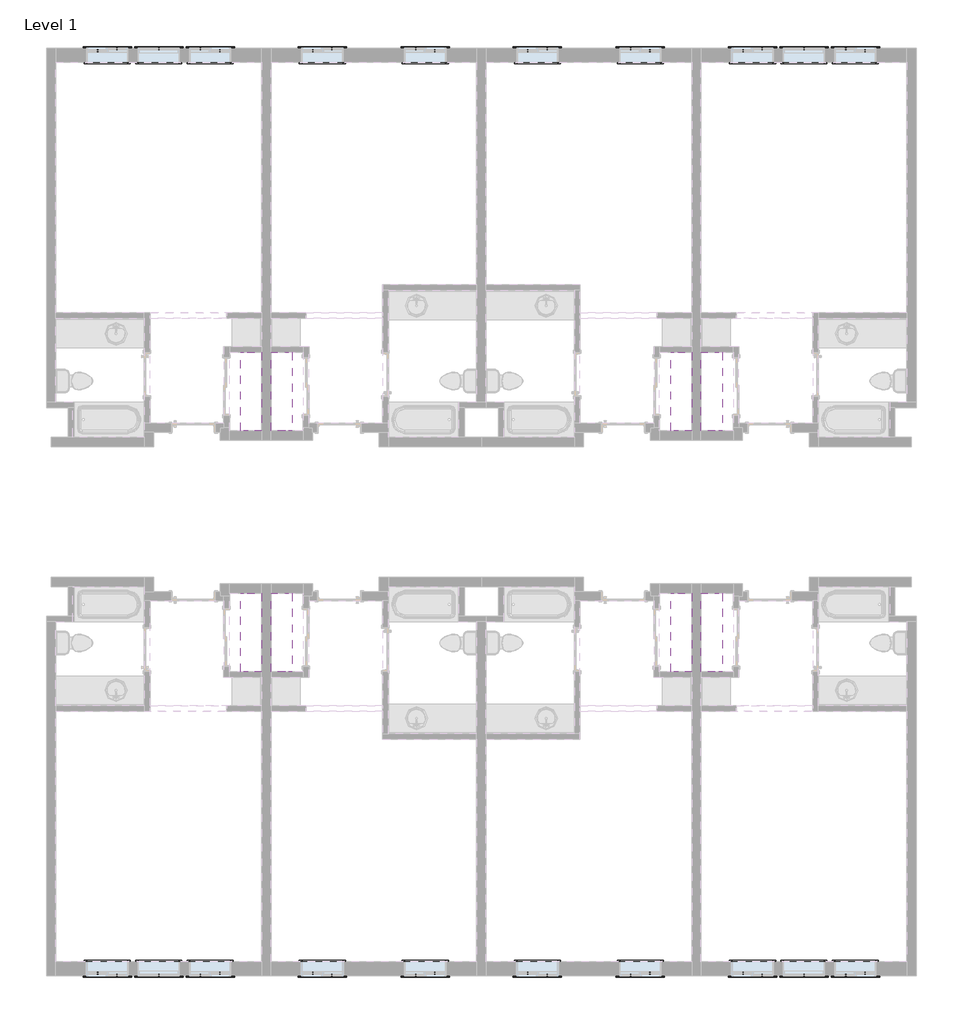
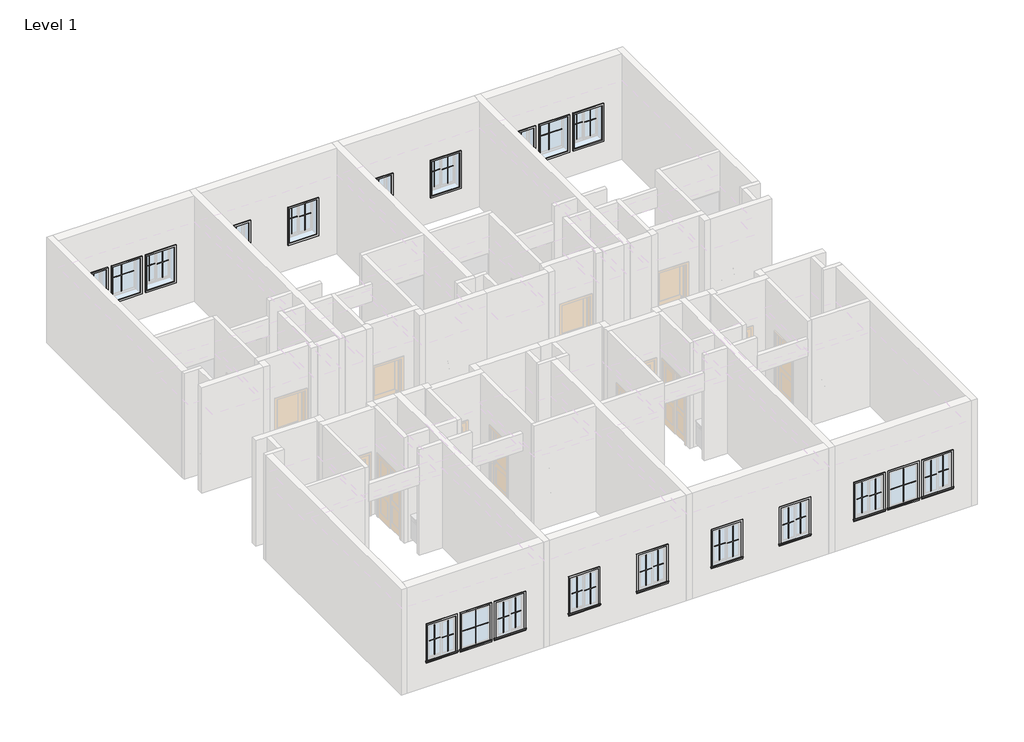
# One storey, part 5 of 5: 84 proxies.
"""IFC4 building model written with IfcOpenShell, lengths in millimetres."""

import ifcopenshell
import ifcopenshell.guid

model = None  # the IFC model being written
_history = None  # IfcOwnerHistory: only IFC2X3 demands one
_inside = {}  # id of a spatial element -> (the spatial element, [elements in it])
_under = {}  # id of a project, library or spatial element -> (it, [spatial elements below it])
_declared = {}  # id of a project -> (the project, [libraries it declares])
_typed = {}  # id of a type object -> (the type object, [elements of that type])
_made_of = {}  # id of a material, layer set ... -> (it, [elements and type objects made of it])


def new_model(schema):
    """Start an empty IFC model of exactly this schema.

    Asked for "IFC4X3", IfcOpenShell would pick the latest addendum, in which some entities
    have other attributes; the version numbers below select the first issue.
    IFC2X3 requires an IfcOwnerHistory on every rooted entity: one is made here for all.
    """
    global model, _history
    if schema == "IFC4X3":
        model = ifcopenshell.file(schema_version=(4, 3, 0, 0))
    else:
        model = ifcopenshell.file(schema=schema)
    _inside.clear()
    _under.clear()
    _declared.clear()
    _typed.clear()
    _made_of.clear()
    _history = None
    if model.schema == "IFC2X3":
        org = make("IfcOrganization", Name="unknown")
        user = make(
            "IfcPersonAndOrganization",
            ThePerson=make("IfcPerson", FamilyName="unknown"),
            TheOrganization=org,
        )
        app = make(
            "IfcApplication",
            ApplicationDeveloper=org,
            Version="unknown",
            ApplicationFullName="unknown",
            ApplicationIdentifier="unknown",
        )
        _history = make(
            "IfcOwnerHistory",
            OwningUser=user,
            OwningApplication=app,
            ChangeAction="ADDED",
            CreationDate=0,
        )
    return model


def make(cls, **values):
    """One entity of the class cls with the attributes given. An attribute that is None is left unset."""
    return model.create_entity(
        cls, **{name: value for name, value in values.items() if value is not None}
    )


def rooted(cls, **values):
    """An entity with a GlobalId (a new one), such as an element, a storey or a relation."""
    return make(cls, GlobalId=ifcopenshell.guid.new(), OwnerHistory=_history, **values)


def si_unit(unit_type, name, prefix=None):
    """IfcSIUnit, for example si_unit("LENGTHUNIT", "METRE", prefix="MILLI")."""
    return make("IfcSIUnit", UnitType=unit_type, Prefix=prefix, Name=name)


def assignment(units):
    """IfcUnitAssignment: the units of a project."""
    return None if units is None else make("IfcUnitAssignment", Units=units)


def point(xyz):
    """IfcCartesianPoint."""
    return None if xyz is None else make("IfcCartesianPoint", Coordinates=xyz)


def direction(xyz):
    """IfcDirection."""
    return None if xyz is None else make("IfcDirection", DirectionRatios=xyz)


def frame(location, z_axis=None, x_axis=None):
    """IfcAxis2Placement3D, a coordinate frame: its origin and axes. An axis left out is left unset."""
    return make(
        "IfcAxis2Placement3D",
        Location=point(location),
        Axis=direction(z_axis),
        RefDirection=direction(x_axis),
    )


def frame_2d(location, x_axis=None):
    """IfcAxis2Placement2D, a coordinate frame in the plane: its origin and x axis."""
    return make(
        "IfcAxis2Placement2D", Location=point(location), RefDirection=direction(x_axis)
    )


def origin():
    """The frame at (0, 0, 0) with its axes left unset."""
    return frame((0.0, 0.0, 0.0))


def origin_with_axes():
    """The frame at (0, 0, 0) with the z axis (0, 0, 1) and the x axis (1, 0, 0) written out."""
    return frame((0.0, 0.0, 0.0), z_axis=(0.0, 0.0, 1.0), x_axis=(1.0, 0.0, 0.0))


def place(relative_to, where):
    """IfcLocalPlacement: puts the frame where relative to a parent placement (None: the world)."""
    return make(
        "IfcLocalPlacement", PlacementRelTo=relative_to, RelativePlacement=where
    )


def context(
    kind, dimensions, precision=None, world=None, true_north=None, identifier=None
):
    """IfcGeometricRepresentationContext, for example the 3D "Model" context."""
    return make(
        "IfcGeometricRepresentationContext",
        ContextIdentifier=identifier,
        ContextType=kind,
        CoordinateSpaceDimension=dimensions,
        Precision=precision,
        WorldCoordinateSystem=world,
        TrueNorth=true_north,
    )


def project(units=None, contexts=None):
    """IfcProject with its units and contexts."""
    return rooted(
        "IfcProject",
        Name="project",
        RepresentationContexts=contexts,
        UnitsInContext=assignment(units),
    )


def spatial(cls, under=None, at=None, **own):
    """A site, building, storey or space (cls), placed at a placement, below another one or the project."""
    s = rooted(cls, ObjectPlacement=at, **own)
    if under is not None:
        _under.setdefault(under.id(), (under, []))[1].append(s)
    return s


def polyline(points):
    """IfcPolyline through the points."""
    return make("IfcPolyline", Points=[point(p) for p in points])


def circle_curve(where, radius):
    """IfcCircle in the frame where."""
    return make("IfcCircle", Position=where, Radius=radius)


def trimmed(basis, trim1, trim2, sense, master):
    """IfcTrimmedCurve: the piece of a basis curve between two trims."""
    return make(
        "IfcTrimmedCurve",
        BasisCurve=basis,
        Trim1=trim1,
        Trim2=trim2,
        SenseAgreement=sense,
        MasterRepresentation=master,
    )


def segment(curve, same_sense, transition):
    """IfcCompositeCurveSegment."""
    return make(
        "IfcCompositeCurveSegment",
        Transition=transition,
        SameSense=same_sense,
        ParentCurve=curve,
    )


def composite_curve(segments, self_intersect=None):
    """IfcCompositeCurve: segments joined end to end."""
    return make("IfcCompositeCurve", Segments=segments, SelfIntersect=self_intersect)


def outline(outer, holes=None, kind="AREA"):
    """IfcArbitraryClosedProfileDef: a profile drawn as a closed curve; with holes, ...WithVoids."""
    if holes is None:
        return make("IfcArbitraryClosedProfileDef", ProfileType=kind, OuterCurve=outer)
    return make(
        "IfcArbitraryProfileDefWithVoids",
        ProfileType=kind,
        OuterCurve=outer,
        InnerCurves=holes,
    )


def extrude(swept, where, along, depth):
    """IfcExtrudedAreaSolid: the profile swept, set in the frame where, extruded along a direction by depth."""
    return make(
        "IfcExtrudedAreaSolid",
        SweptArea=swept,
        Position=where,
        ExtrudedDirection=direction(along),
        Depth=depth,
    )


def shape(context_of_items, identifier, shape_type, items):
    """IfcShapeRepresentation: the items that make up one representation, for example the "Body"."""
    return make(
        "IfcShapeRepresentation",
        ContextOfItems=context_of_items,
        RepresentationIdentifier=identifier,
        RepresentationType=shape_type,
        Items=items,
    )


def source(mapping_origin, context_of_items, identifier, shape_type, items):
    """IfcRepresentationMap: a shape defined once, which mapped items show again and again."""
    return make(
        "IfcRepresentationMap",
        MappingOrigin=mapping_origin,
        MappedRepresentation=shape(context_of_items, identifier, shape_type, items),
    )


def transform(
    local_origin,
    x_axis=None,
    y_axis=None,
    z_axis=None,
    scale=None,
    scale2=None,
    scale3=None,
    uniform=True,
):
    """IfcCartesianTransformationOperator3D, or its non-uniform kind. x_axis, y_axis, z_axis: its Axis1, 2, 3."""
    if uniform:
        return make(
            "IfcCartesianTransformationOperator3D",
            Axis1=direction(x_axis),
            Axis2=direction(y_axis),
            LocalOrigin=point(local_origin),
            Scale=scale,
            Axis3=direction(z_axis),
        )
    return make(
        "IfcCartesianTransformationOperator3DnonUniform",
        Axis1=direction(x_axis),
        Axis2=direction(y_axis),
        LocalOrigin=point(local_origin),
        Scale=scale,
        Axis3=direction(z_axis),
        Scale2=scale2,
        Scale3=scale3,
    )


def mapped(mapping_source, mapping_target):
    """IfcMappedItem: shows the shape of a source again, moved by a transform."""
    return make(
        "IfcMappedItem", MappingSource=mapping_source, MappingTarget=mapping_target
    )


def made_of(thing, what):
    """Note that an element or type object is made of a material, layer set ...; save() writes the relation."""
    if what is not None:
        _made_of.setdefault(what.id(), (what, []))[1].append(thing)
    return thing


def element(
    cls,
    number,
    at=None,
    inside=None,
    cuts=None,
    type_object=None,
    material=None,
    context=None,
    identifier="Body",
    shape_type=None,
    held_by="IfcProductDefinitionShape",
    body=None,
    shapes=None,
    **own,
):
    """One element of the class cls, such as IfcWall. Its Tag is "e" and its number.

    at: its placement. inside: the storey or other place that contains it. cuts: it is an
    opening in that element (IfcRelVoidsElement). A single representation is given by context,
    identifier, shape_type and body (its items); several are given by shapes. held_by: the class
    of the entity that holds the representations. save() writes the other relations.
    """
    e = rooted(cls, Tag="e%d" % number, ObjectPlacement=at, **own)
    if body is not None:
        shapes = [shape(context, identifier, shape_type, body)]
    if shapes is not None:
        e.Representation = make(held_by, Representations=shapes)
    if inside is not None:
        _inside.setdefault(inside.id(), (inside, []))[1].append(e)
    if cuts is not None:
        rooted(
            "IfcRelVoidsElement", RelatingBuildingElement=cuts, RelatedOpeningElement=e
        )
    if type_object is not None:
        _typed.setdefault(type_object.id(), (type_object, []))[1].append(e)
    return made_of(e, material)


def aggregate(whole, parts):
    """IfcRelAggregates: a whole, such as a stair, and the parts it consists of."""
    return rooted("IfcRelAggregates", RelatingObject=whole, RelatedObjects=parts)


def save(model, path):
    """Write the relations noted so far, then the file.

    IfcRelAggregates (storeys below a building ...), IfcRelContainedInSpatialStructure (elements
    in a storey), IfcRelDefinesByType, IfcRelAssociatesMaterial and IfcRelDeclares: one each for
    every whole, place, type object, material and project.
    """
    for whole, parts in _under.values():
        aggregate(whole, parts)
    for where, things in _inside.values():
        rooted(
            "IfcRelContainedInSpatialStructure",
            RelatedElements=things,
            RelatingStructure=where,
        )
    for kind, things in _typed.values():
        rooted("IfcRelDefinesByType", RelatedObjects=things, RelatingType=kind)
    for what, things in _made_of.values():
        rooted("IfcRelAssociatesMaterial", RelatedObjects=things, RelatingMaterial=what)
    for by, libraries in _declared.values():
        rooted("IfcRelDeclares", RelatingContext=by, RelatedDefinitions=libraries)
    model.write(path)


def proxy_eadc3ce0(model_context):
    return source(origin(), model_context, "Body", "SweptSolid", [
        extrude(outline(composite_curve([segment(trimmed(circle_curve(frame_2d((-304.8, 1676.4)), 9.525), [point((-314.325, 1676.4))], [point((-295.275, 1676.4))], False, "CARTESIAN"), True, "CONTINUOUS"), segment(trimmed(circle_curve(frame_2d((-304.8, 1676.4)), 9.525), [point((-295.275, 1676.4))], [point((-314.325, 1676.4))], False, "CARTESIAN"), True, "CONTINUOUS")], self_intersect=False)), frame((0.0, 0.0, 0.0), z_axis=(1.0, 0.0, 0.0), x_axis=(0.0, 1.0, 0.0)), (0.0, 0.0, 1.0), 1701.8),
        extrude(outline(polyline([(1701.8, 0.0), (1701.8, -457.2), (0.0, -457.2), (0.0, 0.0), (1701.8, 0.0)])), frame((0.0, 0.0, 1809.75), z_axis=(0.0, 0.0, 1.0), x_axis=(1.0, 0.0, 0.0)), (0.0, 0.0, 1.0), 19.05),
    ])


def proxy_9baf1220(model_context):
    return source(origin(), model_context, "Body", "SweptSolid", [
        extrude(outline(composite_curve([segment(trimmed(circle_curve(frame_2d((304.8, 1676.4)), 9.525), [point((314.325, 1676.4))], [point((295.275, 1676.4))], False, "CARTESIAN"), True, "CONTINUOUS"), segment(trimmed(circle_curve(frame_2d((304.8, 1676.4)), 9.525), [point((295.275, 1676.4))], [point((314.325, 1676.4))], False, "CARTESIAN"), True, "CONTINUOUS")], self_intersect=False)), frame((0.0, 0.0, 0.0), z_axis=(1.0, 0.0, 0.0), x_axis=(0.0, 1.0, 0.0)), (0.0, 0.0, 1.0), 1701.8),
        extrude(outline(polyline([(1701.8, 0.0), (0.0, 0.0), (0.0, 457.2), (1701.8, 457.2), (1701.8, 0.0)])), frame((0.0, 0.0, 1809.75), z_axis=(0.0, 0.0, 1.0), x_axis=(1.0, 0.0, 0.0)), (0.0, 0.0, 1.0), 19.05),
    ])


def muntin_pattern_2x2_muntin_pattern_2x2_0b2f62cf(model_context):
    return source(origin(), model_context, "Body", "SweptSolid", [
        extrude(outline(polyline([(577.85, -6.35), (577.85, -419.1), (565.15, -419.1), (565.15, -6.35), (0.0, -6.35), (0.0, 6.35), (565.15, 6.35), (565.15, 419.1), (577.85, 419.1), (577.85, 6.35), (1143.0, 6.35), (1143.0, -6.35), (577.85, -6.35)])), frame((0.0, -22.225, 0.0), z_axis=(0.0, 1.0, 0.0), x_axis=(0.0, 0.0, 1.0)), (0.0, 0.0, 1.0), 12.7),
        extrude(outline(polyline([(577.85, -6.35), (577.85, -419.1), (565.15, -419.1), (565.15, -6.35), (0.0, -6.35), (0.0, 6.35), (565.15, 6.35), (565.15, 419.1), (577.85, 419.1), (577.85, 6.35), (1143.0, 6.35), (1143.0, -6.35), (577.85, -6.35)])), frame((0.0, 9.525, 0.0), z_axis=(0.0, 1.0, 0.0), x_axis=(0.0, 0.0, 1.0)), (0.0, 0.0, 1.0), 12.7),
    ])


def muntin_pattern_2x2_muntin_pattern_2x2_764e8cbb(model_context):
    return source(origin(), model_context, "Body", "SweptSolid", [
        extrude(outline(polyline([(542.925, -6.35), (542.925, -185.7375), (530.225, -185.7375), (530.225, -6.35), (0.0, -6.35), (0.0, 6.35), (530.225, 6.35), (530.225, 185.7375), (542.925, 185.7375), (542.925, 6.35), (1073.15, 6.35), (1073.15, -6.35), (542.925, -6.35)])), frame((0.0, -22.225, 0.0), z_axis=(0.0, 1.0, 0.0), x_axis=(0.0, 0.0, 1.0)), (0.0, 0.0, 1.0), 12.7),
        extrude(outline(polyline([(542.925, -6.35), (542.925, -185.7375), (530.225, -185.7375), (530.225, -6.35), (0.0, -6.35), (0.0, 6.35), (530.225, 6.35), (530.225, 185.7375), (542.925, 185.7375), (542.925, 6.35), (1073.15, 6.35), (1073.15, -6.35), (542.925, -6.35)])), frame((0.0, 9.525, 0.0), z_axis=(0.0, 1.0, 0.0), x_axis=(0.0, 0.0, 1.0)), (0.0, 0.0, 1.0), 12.7),
    ])


def muntin_pattern_2x2_muntin_pattern_2x2_daa3f335(model_context):
    return source(origin(), model_context, "Body", "SweptSolid", [
        extrude(outline(polyline([(542.925, -6.35), (542.925, -185.7375), (530.225, -185.7375), (530.225, -6.35), (0.0, -6.35), (0.0, 6.35), (530.225, 6.35), (530.225, 185.7375), (542.925, 185.7375), (542.925, 6.35), (1073.15, 6.35), (1073.15, -6.35), (542.925, -6.35)])), frame((0.0, 9.525, 0.0), z_axis=(0.0, 1.0, 0.0), x_axis=(0.0, 0.0, 1.0)), (0.0, 0.0, 1.0), 12.7),
        extrude(outline(polyline([(542.925, -6.35), (542.925, -185.7375), (530.225, -185.7375), (530.225, -6.35), (0.0, -6.35), (0.0, 6.35), (530.225, 6.35), (530.225, 185.7375), (542.925, 185.7375), (542.925, 6.35), (1073.15, 6.35), (1073.15, -6.35), (542.925, -6.35)])), frame((0.0, -22.225, 0.0), z_axis=(0.0, 1.0, 0.0), x_axis=(0.0, 0.0, 1.0)), (0.0, 0.0, 1.0), 12.7),
    ])


def muntin_pattern_2x2_muntin_pattern_2x2_a23de983(model_context):
    return source(origin(), model_context, "Body", "SweptSolid", [
        extrude(outline(polyline([(577.85, -6.35), (577.85, -419.1), (565.15, -419.1), (565.15, -6.35), (0.0, -6.35), (0.0, 6.35), (565.15, 6.35), (565.15, 419.1), (577.85, 419.1), (577.85, 6.35), (1143.0, 6.35), (1143.0, -6.35), (577.85, -6.35)])), frame((0.0, 9.525, 0.0), z_axis=(0.0, 1.0, 0.0), x_axis=(0.0, 0.0, 1.0)), (0.0, 0.0, 1.0), 12.7),
        extrude(outline(polyline([(577.85, -6.35), (577.85, -419.1), (565.15, -419.1), (565.15, -6.35), (0.0, -6.35), (0.0, 6.35), (565.15, 6.35), (565.15, 419.1), (577.85, 419.1), (577.85, 6.35), (1143.0, 6.35), (1143.0, -6.35), (577.85, -6.35)])), frame((0.0, -22.225, 0.0), z_axis=(0.0, 1.0, 0.0), x_axis=(0.0, 0.0, 1.0)), (0.0, 0.0, 1.0), 12.7),
    ])


def trim_window_exterior_flat_with_sill_e4b28ec3(model_context):
    return source(origin(), model_context, "Body", "SweptSolid", [
        extrude(outline(polyline([(514.35, -1241.3823709), (514.35, -1298.5323709), (-514.35, -1298.5323709), (-514.35, -1241.3823709), (514.35, -1241.3823709)])), origin_with_axes(), (0.0, 0.0, 1.0), 19.05),
        extrude(outline(polyline([(-1250.95, 38.1), (-1221.6580645, 38.1), (-1219.2, 19.05), (-1219.2, 0.0), (-1241.3823709, 0.0), (-1241.3823709, 19.05), (-1250.95, 19.05), (-1250.95, 38.1)])), frame((-527.05, 0.0, 0.0), z_axis=(1.0, 0.0, 0.0), x_axis=(0.0, 1.0, 0.0)), (0.0, 0.0, 1.0), 1054.1),
        extrude(outline(polyline([(-514.35, 57.15), (514.35, 57.15), (514.35, -1219.2), (457.2, -1219.2), (457.2, 0.0), (-457.2, 0.0), (-457.2, -1219.2), (-514.35, -1219.2), (-514.35, 57.15)])), origin_with_axes(), (0.0, 0.0, 1.0), 19.05),
    ])


def trim_window_exterior_flat_with_sill_80371c4b(model_context):
    return source(origin(), model_context, "Body", "SweptSolid", [
        extrude(outline(polyline([(514.35, 1241.3823709), (-514.35, 1241.3823709), (-514.35, 1298.5323709), (514.35, 1298.5323709), (514.35, 1241.3823709)])), origin_with_axes(), (0.0, 0.0, 1.0), 19.05),
        extrude(outline(polyline([(1250.95, 38.1), (1250.95, 19.05), (1241.3823709, 19.05), (1241.3823709, 0.0), (1219.2, 0.0), (1219.2, 19.05), (1221.6580645, 38.1), (1250.95, 38.1)])), frame((-527.05, 0.0, 0.0), z_axis=(1.0, 0.0, 0.0), x_axis=(0.0, 1.0, 0.0)), (0.0, 0.0, 1.0), 1054.1),
        extrude(outline(polyline([(-514.35, -57.15), (-514.35, 1219.2), (-457.2, 1219.2), (-457.2, 0.0), (457.2, 0.0), (457.2, 1219.2), (514.35, 1219.2), (514.35, -57.15), (-514.35, -57.15)])), origin_with_axes(), (0.0, 0.0, 1.0), 19.05),
    ])


def trim_window_interior_flat_picture_frame_39ff4276(model_context):
    return source(origin(), model_context, "Body", "SweptSolid", [
        extrude(outline(polyline([(501.65, 44.45), (501.65, -1263.65), (-501.65, -1263.65), (-501.65, 44.45), (501.65, 44.45)]), holes=[polyline([(444.5, -12.7), (-444.5, -12.7), (-444.5, -1206.5), (444.5, -1206.5), (444.5, -12.7)])]), origin_with_axes(), (0.0, 0.0, 1.0), 31.75),
    ])


def trim_window_interior_flat_picture_frame_c1dcbb6d(model_context):
    return source(origin(), model_context, "Body", "SweptSolid", [
        extrude(outline(polyline([(501.65, -44.45), (-501.65, -44.45), (-501.65, 1263.65), (501.65, 1263.65), (501.65, -44.45)]), holes=[polyline([(444.5, 12.7), (444.5, 1206.5), (-444.5, 1206.5), (-444.5, 12.7), (444.5, 12.7)])]), origin_with_axes(), (0.0, 0.0, 1.0), 31.75),
    ])


model = new_model("IFC4")

# Units and contexts
model_context = context("Model", 3, world=origin())
ifc_project = project(units=[si_unit("LENGTHUNIT", "METRE", prefix="MILLI")], contexts=[model_context])

# Site, building, storey
site = spatial("IfcSite", under=ifc_project)
building = spatial("IfcBuilding", under=site)
storey = spatial("IfcBuildingStorey", under=building, Name="Level 1", Elevation=0.0)

# Proxies
placement = place(None, origin())
proxy_shape = proxy_eadc3ce0(model_context)
element("IfcBuildingElementProxy", 1, Name="Closet Shelf and Pole : 18\" Deep", ObjectType="Closet Shelf and Pole : 18\" Deep", at=placement, inside=storey, context=model_context, shape_type="MappedRepresentation", body=[
    mapped(proxy_shape, transform((-10892.3979403, 8312.6765484, 0.0), x_axis=(0.0, -1.0, 0.0), y_axis=(1.0, 0.0, 0.0), z_axis=(0.0, 0.0, 1.0))),
])
element("IfcBuildingElementProxy", 2, Name="Closet Shelf and Pole : 18\" Deep", ObjectType="Closet Shelf and Pole : 18\" Deep", at=placement, inside=storey, context=model_context, shape_type="MappedRepresentation", body=[
    mapped(proxy_shape, transform((-1341.9979403, 11843.2765484, 0.0), x_axis=(0.0, 1.0, 0.0), y_axis=(-1.0, 0.0, 0.0), z_axis=(0.0, 0.0, 1.0))),
])
element("IfcBuildingElementProxy", 3, Name="Closet Shelf and Pole : 18\" Deep", ObjectType="Closet Shelf and Pole : 18\" Deep", at=placement, inside=storey, context=model_context, shape_type="MappedRepresentation", body=[
    mapped(proxy_shape, transform((-10689.1979403, 11843.2765484, 0.0), x_axis=(0.0, 1.0, 0.0), y_axis=(-1.0, 0.0, 0.0), z_axis=(0.0, 0.0, 1.0))),
])
element("IfcBuildingElementProxy", 4, Name="Closet Shelf and Pole : 18\" Deep", ObjectType="Closet Shelf and Pole : 18\" Deep", at=placement, inside=storey, context=model_context, shape_type="MappedRepresentation", body=[
    mapped(proxy_shape, transform((-1545.1979403, 8312.6765484, 0.0), x_axis=(0.0, -1.0, 0.0), y_axis=(1.0, 0.0, 0.0), z_axis=(0.0, 0.0, 1.0))),
])
proxy_2_shape = proxy_9baf1220(model_context)
element("IfcBuildingElementProxy", 5, Name="Closet Shelf and Pole : 18\" Deep", ObjectType="Closet Shelf and Pole : 18\" Deep", at=placement, inside=storey, context=model_context, shape_type="MappedRepresentation", body=[
    mapped(proxy_2_shape, transform((-10892.3979403, 11843.2765484, 0.0), x_axis=(0.0, 1.0, 0.0), y_axis=(-1.0, 0.0, 0.0), z_axis=(0.0, 0.0, 1.0))),
])
element("IfcBuildingElementProxy", 6, Name="Closet Shelf and Pole : 18\" Deep", ObjectType="Closet Shelf and Pole : 18\" Deep", at=placement, inside=storey, context=model_context, shape_type="MappedRepresentation", body=[
    mapped(proxy_2_shape, transform((-1341.9979403, 8312.6765484, 0.0), x_axis=(0.0, -1.0, 0.0), y_axis=(1.0, 0.0, 0.0), z_axis=(0.0, 0.0, 1.0))),
])
element("IfcBuildingElementProxy", 7, Name="Closet Shelf and Pole : 18\" Deep", ObjectType="Closet Shelf and Pole : 18\" Deep", at=placement, inside=storey, context=model_context, shape_type="MappedRepresentation", body=[
    mapped(proxy_2_shape, transform((-10689.1979403, 8312.6765484, 0.0), x_axis=(0.0, -1.0, 0.0), y_axis=(1.0, 0.0, 0.0), z_axis=(0.0, 0.0, 1.0))),
])
element("IfcBuildingElementProxy", 8, Name="Closet Shelf and Pole : 18\" Deep", ObjectType="Closet Shelf and Pole : 18\" Deep", at=placement, inside=storey, context=model_context, shape_type="MappedRepresentation", body=[
    mapped(proxy_2_shape, transform((-1545.1979403, 11843.2765484, 0.0), x_axis=(0.0, 1.0, 0.0), y_axis=(-1.0, 0.0, 0.0), z_axis=(0.0, 0.0, 1.0))),
])
muntin_pattern_2x2_muntin_pattern_2x2_shape = muntin_pattern_2x2_muntin_pattern_2x2_0b2f62cf(model_context)
element("IfcBuildingElementProxy", 9, Name="Muntin Pattern_2x2 : Muntin Pattern_2x2", ObjectType="Muntin Pattern_2x2 : Muntin Pattern_2x2", at=placement, inside=storey, context=model_context, shape_type="MappedRepresentation", body=[
    mapped(muntin_pattern_2x2_muntin_pattern_2x2_shape, transform((-13127.5979403, 16.4015484, 952.5), x_axis=(1.0, 0.0, 0.0), y_axis=(0.0, 1.0, 0.0), z_axis=(0.0, 0.0, 1.0))),
])
element("IfcBuildingElementProxy", 10, Name="Muntin Pattern_2x2 : Muntin Pattern_2x2", ObjectType="Muntin Pattern_2x2 : Muntin Pattern_2x2", at=placement, inside=storey, context=model_context, shape_type="MappedRepresentation", body=[
    mapped(muntin_pattern_2x2_muntin_pattern_2x2_shape, transform((893.2020597, 20139.5515484, 952.5), x_axis=(-1.0, 0.0, 0.0), y_axis=(0.0, -1.0, 0.0), z_axis=(0.0, 0.0, 1.0))),
])
muntin_pattern_2x2_muntin_pattern_2x2_2_shape = muntin_pattern_2x2_muntin_pattern_2x2_764e8cbb(model_context)
element("IfcBuildingElementProxy", 11, Name="Muntin Pattern_2x2 : Muntin Pattern_2x2", ObjectType="Muntin Pattern_2x2 : Muntin Pattern_2x2", at=placement, inside=storey, context=model_context, shape_type="MappedRepresentation", body=[
    mapped(muntin_pattern_2x2_muntin_pattern_2x2_2_shape, transform((-11802.0354403, 60.8515484, 996.95), x_axis=(1.0, 0.0, 0.0), y_axis=(0.0, 1.0, 0.0), z_axis=(0.0, 0.0, 1.0))),
])
element("IfcBuildingElementProxy", 12, Name="Muntin Pattern_2x2 : Muntin Pattern_2x2", ObjectType="Muntin Pattern_2x2 : Muntin Pattern_2x2", at=placement, inside=storey, context=model_context, shape_type="MappedRepresentation", body=[
    mapped(muntin_pattern_2x2_muntin_pattern_2x2_2_shape, transform((-12217.9604403, 16.4015484, 996.95), x_axis=(1.0, 0.0, 0.0), y_axis=(0.0, 1.0, 0.0), z_axis=(0.0, 0.0, 1.0))),
])
element("IfcBuildingElementProxy", 13, Name="Muntin Pattern_2x2 : Muntin Pattern_2x2", ObjectType="Muntin Pattern_2x2 : Muntin Pattern_2x2", at=placement, inside=storey, context=model_context, shape_type="MappedRepresentation", body=[
    mapped(muntin_pattern_2x2_muntin_pattern_2x2_2_shape, transform((-14453.1604403, 20095.1015484, 996.95), x_axis=(-1.0, 0.0, 0.0), y_axis=(0.0, -1.0, 0.0), z_axis=(0.0, 0.0, 1.0))),
])
element("IfcBuildingElementProxy", 14, Name="Muntin Pattern_2x2 : Muntin Pattern_2x2", ObjectType="Muntin Pattern_2x2 : Muntin Pattern_2x2", at=placement, inside=storey, context=model_context, shape_type="MappedRepresentation", body=[
    mapped(muntin_pattern_2x2_muntin_pattern_2x2_2_shape, transform((-14037.2354403, 20139.5515484, 996.95), x_axis=(-1.0, 0.0, 0.0), y_axis=(0.0, -1.0, 0.0), z_axis=(0.0, 0.0, 1.0))),
])
element("IfcBuildingElementProxy", 15, Name="Muntin Pattern_2x2 : Muntin Pattern_2x2", ObjectType="Muntin Pattern_2x2 : Muntin Pattern_2x2", at=placement, inside=storey, context=model_context, shape_type="MappedRepresentation", body=[
    mapped(muntin_pattern_2x2_muntin_pattern_2x2_2_shape, transform((2218.7645597, 60.8515484, 996.95), x_axis=(1.0, 0.0, 0.0), y_axis=(0.0, 1.0, 0.0), z_axis=(0.0, 0.0, 1.0))),
])
element("IfcBuildingElementProxy", 16, Name="Muntin Pattern_2x2 : Muntin Pattern_2x2", ObjectType="Muntin Pattern_2x2 : Muntin Pattern_2x2", at=placement, inside=storey, context=model_context, shape_type="MappedRepresentation", body=[
    mapped(muntin_pattern_2x2_muntin_pattern_2x2_2_shape, transform((1802.8395597, 16.4015484, 996.95), x_axis=(1.0, 0.0, 0.0), y_axis=(0.0, 1.0, 0.0), z_axis=(0.0, 0.0, 1.0))),
])
element("IfcBuildingElementProxy", 17, Name="Muntin Pattern_2x2 : Muntin Pattern_2x2", ObjectType="Muntin Pattern_2x2 : Muntin Pattern_2x2", at=placement, inside=storey, context=model_context, shape_type="MappedRepresentation", body=[
    mapped(muntin_pattern_2x2_muntin_pattern_2x2_2_shape, transform((-432.3604403, 20095.1015484, 996.95), x_axis=(-1.0, 0.0, 0.0), y_axis=(0.0, -1.0, 0.0), z_axis=(0.0, 0.0, 1.0))),
])
element("IfcBuildingElementProxy", 18, Name="Muntin Pattern_2x2 : Muntin Pattern_2x2", ObjectType="Muntin Pattern_2x2 : Muntin Pattern_2x2", at=placement, inside=storey, context=model_context, shape_type="MappedRepresentation", body=[
    mapped(muntin_pattern_2x2_muntin_pattern_2x2_2_shape, transform((-16.4354403, 20139.5515484, 996.95), x_axis=(-1.0, 0.0, 0.0), y_axis=(0.0, -1.0, 0.0), z_axis=(0.0, 0.0, 1.0))),
])
element("IfcBuildingElementProxy", 19, Name="Muntin Pattern_2x2 : Muntin Pattern_2x2", ObjectType="Muntin Pattern_2x2 : Muntin Pattern_2x2", at=placement, inside=storey, context=model_context, shape_type="MappedRepresentation", body=[
    mapped(muntin_pattern_2x2_muntin_pattern_2x2_2_shape, transform((-7128.4354403, 60.8515484, 996.95), x_axis=(1.0, 0.0, 0.0), y_axis=(0.0, 1.0, 0.0), z_axis=(0.0, 0.0, 1.0))),
])
element("IfcBuildingElementProxy", 20, Name="Muntin Pattern_2x2 : Muntin Pattern_2x2", ObjectType="Muntin Pattern_2x2 : Muntin Pattern_2x2", at=placement, inside=storey, context=model_context, shape_type="MappedRepresentation", body=[
    mapped(muntin_pattern_2x2_muntin_pattern_2x2_2_shape, transform((-7544.3604403, 16.4015484, 996.95), x_axis=(1.0, 0.0, 0.0), y_axis=(0.0, 1.0, 0.0), z_axis=(0.0, 0.0, 1.0))),
])
element("IfcBuildingElementProxy", 21, Name="Muntin Pattern_2x2 : Muntin Pattern_2x2", ObjectType="Muntin Pattern_2x2 : Muntin Pattern_2x2", at=placement, inside=storey, context=model_context, shape_type="MappedRepresentation", body=[
    mapped(muntin_pattern_2x2_muntin_pattern_2x2_2_shape, transform((-9779.5604403, 20095.1015484, 996.95), x_axis=(-1.0, 0.0, 0.0), y_axis=(0.0, -1.0, 0.0), z_axis=(0.0, 0.0, 1.0))),
])
element("IfcBuildingElementProxy", 22, Name="Muntin Pattern_2x2 : Muntin Pattern_2x2", ObjectType="Muntin Pattern_2x2 : Muntin Pattern_2x2", at=placement, inside=storey, context=model_context, shape_type="MappedRepresentation", body=[
    mapped(muntin_pattern_2x2_muntin_pattern_2x2_2_shape, transform((-9363.6354403, 20139.5515484, 996.95), x_axis=(-1.0, 0.0, 0.0), y_axis=(0.0, -1.0, 0.0), z_axis=(0.0, 0.0, 1.0))),
])
element("IfcBuildingElementProxy", 23, Name="Muntin Pattern_2x2 : Muntin Pattern_2x2", ObjectType="Muntin Pattern_2x2 : Muntin Pattern_2x2", at=placement, inside=storey, context=model_context, shape_type="MappedRepresentation", body=[
    mapped(muntin_pattern_2x2_muntin_pattern_2x2_2_shape, transform((-2454.8354403, 60.8515484, 996.95), x_axis=(1.0, 0.0, 0.0), y_axis=(0.0, 1.0, 0.0), z_axis=(0.0, 0.0, 1.0))),
])
element("IfcBuildingElementProxy", 24, Name="Muntin Pattern_2x2 : Muntin Pattern_2x2", ObjectType="Muntin Pattern_2x2 : Muntin Pattern_2x2", at=placement, inside=storey, context=model_context, shape_type="MappedRepresentation", body=[
    mapped(muntin_pattern_2x2_muntin_pattern_2x2_2_shape, transform((-2870.7604403, 16.4015484, 996.95), x_axis=(1.0, 0.0, 0.0), y_axis=(0.0, 1.0, 0.0), z_axis=(0.0, 0.0, 1.0))),
])
element("IfcBuildingElementProxy", 25, Name="Muntin Pattern_2x2 : Muntin Pattern_2x2", ObjectType="Muntin Pattern_2x2 : Muntin Pattern_2x2", at=placement, inside=storey, context=model_context, shape_type="MappedRepresentation", body=[
    mapped(muntin_pattern_2x2_muntin_pattern_2x2_2_shape, transform((-5105.9604403, 20095.1015484, 996.95), x_axis=(-1.0, 0.0, 0.0), y_axis=(0.0, -1.0, 0.0), z_axis=(0.0, 0.0, 1.0))),
])
element("IfcBuildingElementProxy", 26, Name="Muntin Pattern_2x2 : Muntin Pattern_2x2", ObjectType="Muntin Pattern_2x2 : Muntin Pattern_2x2", at=placement, inside=storey, context=model_context, shape_type="MappedRepresentation", body=[
    mapped(muntin_pattern_2x2_muntin_pattern_2x2_2_shape, transform((-4690.0354403, 20139.5515484, 996.95), x_axis=(-1.0, 0.0, 0.0), y_axis=(0.0, -1.0, 0.0), z_axis=(0.0, 0.0, 1.0))),
])
muntin_pattern_2x2_muntin_pattern_2x2_3_shape = muntin_pattern_2x2_muntin_pattern_2x2_daa3f335(model_context)
element("IfcBuildingElementProxy", 27, Name="Muntin Pattern_2x2 : Muntin Pattern_2x2", ObjectType="Muntin Pattern_2x2 : Muntin Pattern_2x2", at=placement, inside=storey, context=model_context, shape_type="MappedRepresentation", body=[
    mapped(muntin_pattern_2x2_muntin_pattern_2x2_3_shape, transform((-14453.1604403, 60.8515484, 996.95), x_axis=(-1.0, 0.0, 0.0), y_axis=(0.0, -1.0, 0.0), z_axis=(0.0, 0.0, 1.0))),
])
element("IfcBuildingElementProxy", 28, Name="Muntin Pattern_2x2 : Muntin Pattern_2x2", ObjectType="Muntin Pattern_2x2 : Muntin Pattern_2x2", at=placement, inside=storey, context=model_context, shape_type="MappedRepresentation", body=[
    mapped(muntin_pattern_2x2_muntin_pattern_2x2_3_shape, transform((-14037.2354403, 16.4015484, 996.95), x_axis=(-1.0, 0.0, 0.0), y_axis=(0.0, -1.0, 0.0), z_axis=(0.0, 0.0, 1.0))),
])
element("IfcBuildingElementProxy", 29, Name="Muntin Pattern_2x2 : Muntin Pattern_2x2", ObjectType="Muntin Pattern_2x2 : Muntin Pattern_2x2", at=placement, inside=storey, context=model_context, shape_type="MappedRepresentation", body=[
    mapped(muntin_pattern_2x2_muntin_pattern_2x2_3_shape, transform((-11802.0354403, 20095.1015484, 996.95), x_axis=(1.0, 0.0, 0.0), y_axis=(0.0, 1.0, 0.0), z_axis=(0.0, 0.0, 1.0))),
])
element("IfcBuildingElementProxy", 30, Name="Muntin Pattern_2x2 : Muntin Pattern_2x2", ObjectType="Muntin Pattern_2x2 : Muntin Pattern_2x2", at=placement, inside=storey, context=model_context, shape_type="MappedRepresentation", body=[
    mapped(muntin_pattern_2x2_muntin_pattern_2x2_3_shape, transform((-12217.9604403, 20139.5515484, 996.95), x_axis=(1.0, 0.0, 0.0), y_axis=(0.0, 1.0, 0.0), z_axis=(0.0, 0.0, 1.0))),
])
element("IfcBuildingElementProxy", 31, Name="Muntin Pattern_2x2 : Muntin Pattern_2x2", ObjectType="Muntin Pattern_2x2 : Muntin Pattern_2x2", at=placement, inside=storey, context=model_context, shape_type="MappedRepresentation", body=[
    mapped(muntin_pattern_2x2_muntin_pattern_2x2_3_shape, transform((-432.3604403, 60.8515484, 996.95), x_axis=(-1.0, 0.0, 0.0), y_axis=(0.0, -1.0, 0.0), z_axis=(0.0, 0.0, 1.0))),
])
element("IfcBuildingElementProxy", 32, Name="Muntin Pattern_2x2 : Muntin Pattern_2x2", ObjectType="Muntin Pattern_2x2 : Muntin Pattern_2x2", at=placement, inside=storey, context=model_context, shape_type="MappedRepresentation", body=[
    mapped(muntin_pattern_2x2_muntin_pattern_2x2_3_shape, transform((-16.4354403, 16.4015484, 996.95), x_axis=(-1.0, 0.0, 0.0), y_axis=(0.0, -1.0, 0.0), z_axis=(0.0, 0.0, 1.0))),
])
element("IfcBuildingElementProxy", 33, Name="Muntin Pattern_2x2 : Muntin Pattern_2x2", ObjectType="Muntin Pattern_2x2 : Muntin Pattern_2x2", at=placement, inside=storey, context=model_context, shape_type="MappedRepresentation", body=[
    mapped(muntin_pattern_2x2_muntin_pattern_2x2_3_shape, transform((2218.7645597, 20095.1015484, 996.95), x_axis=(1.0, 0.0, 0.0), y_axis=(0.0, 1.0, 0.0), z_axis=(0.0, 0.0, 1.0))),
])
element("IfcBuildingElementProxy", 34, Name="Muntin Pattern_2x2 : Muntin Pattern_2x2", ObjectType="Muntin Pattern_2x2 : Muntin Pattern_2x2", at=placement, inside=storey, context=model_context, shape_type="MappedRepresentation", body=[
    mapped(muntin_pattern_2x2_muntin_pattern_2x2_3_shape, transform((1802.8395597, 20139.5515484, 996.95), x_axis=(1.0, 0.0, 0.0), y_axis=(0.0, 1.0, 0.0), z_axis=(0.0, 0.0, 1.0))),
])
element("IfcBuildingElementProxy", 35, Name="Muntin Pattern_2x2 : Muntin Pattern_2x2", ObjectType="Muntin Pattern_2x2 : Muntin Pattern_2x2", at=placement, inside=storey, context=model_context, shape_type="MappedRepresentation", body=[
    mapped(muntin_pattern_2x2_muntin_pattern_2x2_3_shape, transform((-9779.5604403, 60.8515484, 996.95), x_axis=(-1.0, 0.0, 0.0), y_axis=(0.0, -1.0, 0.0), z_axis=(0.0, 0.0, 1.0))),
])
element("IfcBuildingElementProxy", 36, Name="Muntin Pattern_2x2 : Muntin Pattern_2x2", ObjectType="Muntin Pattern_2x2 : Muntin Pattern_2x2", at=placement, inside=storey, context=model_context, shape_type="MappedRepresentation", body=[
    mapped(muntin_pattern_2x2_muntin_pattern_2x2_3_shape, transform((-9363.6354403, 16.4015484, 996.95), x_axis=(-1.0, 0.0, 0.0), y_axis=(0.0, -1.0, 0.0), z_axis=(0.0, 0.0, 1.0))),
])
element("IfcBuildingElementProxy", 37, Name="Muntin Pattern_2x2 : Muntin Pattern_2x2", ObjectType="Muntin Pattern_2x2 : Muntin Pattern_2x2", at=placement, inside=storey, context=model_context, shape_type="MappedRepresentation", body=[
    mapped(muntin_pattern_2x2_muntin_pattern_2x2_3_shape, transform((-7128.4354403, 20095.1015484, 996.95), x_axis=(1.0, 0.0, 0.0), y_axis=(0.0, 1.0, 0.0), z_axis=(0.0, 0.0, 1.0))),
])
element("IfcBuildingElementProxy", 38, Name="Muntin Pattern_2x2 : Muntin Pattern_2x2", ObjectType="Muntin Pattern_2x2 : Muntin Pattern_2x2", at=placement, inside=storey, context=model_context, shape_type="MappedRepresentation", body=[
    mapped(muntin_pattern_2x2_muntin_pattern_2x2_3_shape, transform((-7544.3604403, 20139.5515484, 996.95), x_axis=(1.0, 0.0, 0.0), y_axis=(0.0, 1.0, 0.0), z_axis=(0.0, 0.0, 1.0))),
])
element("IfcBuildingElementProxy", 39, Name="Muntin Pattern_2x2 : Muntin Pattern_2x2", ObjectType="Muntin Pattern_2x2 : Muntin Pattern_2x2", at=placement, inside=storey, context=model_context, shape_type="MappedRepresentation", body=[
    mapped(muntin_pattern_2x2_muntin_pattern_2x2_3_shape, transform((-5105.9604403, 60.8515484, 996.95), x_axis=(-1.0, 0.0, 0.0), y_axis=(0.0, -1.0, 0.0), z_axis=(0.0, 0.0, 1.0))),
])
element("IfcBuildingElementProxy", 40, Name="Muntin Pattern_2x2 : Muntin Pattern_2x2", ObjectType="Muntin Pattern_2x2 : Muntin Pattern_2x2", at=placement, inside=storey, context=model_context, shape_type="MappedRepresentation", body=[
    mapped(muntin_pattern_2x2_muntin_pattern_2x2_3_shape, transform((-4690.0354403, 16.4015484, 996.95), x_axis=(-1.0, 0.0, 0.0), y_axis=(0.0, -1.0, 0.0), z_axis=(0.0, 0.0, 1.0))),
])
element("IfcBuildingElementProxy", 41, Name="Muntin Pattern_2x2 : Muntin Pattern_2x2", ObjectType="Muntin Pattern_2x2 : Muntin Pattern_2x2", at=placement, inside=storey, context=model_context, shape_type="MappedRepresentation", body=[
    mapped(muntin_pattern_2x2_muntin_pattern_2x2_3_shape, transform((-2454.8354403, 20095.1015484, 996.95), x_axis=(1.0, 0.0, 0.0), y_axis=(0.0, 1.0, 0.0), z_axis=(0.0, 0.0, 1.0))),
])
element("IfcBuildingElementProxy", 42, Name="Muntin Pattern_2x2 : Muntin Pattern_2x2", ObjectType="Muntin Pattern_2x2 : Muntin Pattern_2x2", at=placement, inside=storey, context=model_context, shape_type="MappedRepresentation", body=[
    mapped(muntin_pattern_2x2_muntin_pattern_2x2_3_shape, transform((-2870.7604403, 20139.5515484, 996.95), x_axis=(1.0, 0.0, 0.0), y_axis=(0.0, 1.0, 0.0), z_axis=(0.0, 0.0, 1.0))),
])
muntin_pattern_2x2_muntin_pattern_2x2_4_shape = muntin_pattern_2x2_muntin_pattern_2x2_a23de983(model_context)
element("IfcBuildingElementProxy", 43, Name="Muntin Pattern_2x2 : Muntin Pattern_2x2", ObjectType="Muntin Pattern_2x2 : Muntin Pattern_2x2", at=placement, inside=storey, context=model_context, shape_type="MappedRepresentation", body=[
    mapped(muntin_pattern_2x2_muntin_pattern_2x2_4_shape, transform((-13127.5979403, 20139.5515484, 952.5), x_axis=(1.0, 0.0, 0.0), y_axis=(0.0, 1.0, 0.0), z_axis=(0.0, 0.0, 1.0))),
])
element("IfcBuildingElementProxy", 44, Name="Muntin Pattern_2x2 : Muntin Pattern_2x2", ObjectType="Muntin Pattern_2x2 : Muntin Pattern_2x2", at=placement, inside=storey, context=model_context, shape_type="MappedRepresentation", body=[
    mapped(muntin_pattern_2x2_muntin_pattern_2x2_4_shape, transform((893.2020597, 16.4015484, 952.5), x_axis=(-1.0, 0.0, 0.0), y_axis=(0.0, -1.0, 0.0), z_axis=(0.0, 0.0, 1.0))),
])
trim_window_exterior_flat_with_sill_shape = trim_window_exterior_flat_with_sill_e4b28ec3(model_context)
element("IfcBuildingElementProxy", 45, Name="Trim-Window-Exterior-Flat : with Sill", ObjectType="Trim-Window-Exterior-Flat : with Sill", at=placement, inside=storey, context=model_context, shape_type="MappedRepresentation", body=[
    mapped(trim_window_exterior_flat_with_sill_shape, transform((-14245.1979403, 6.8765484, 2133.6), x_axis=(1.0, 0.0, 0.0), y_axis=(0.0, 0.0, 1.0), z_axis=(0.0, -1.0, 0.0))),
])
element("IfcBuildingElementProxy", 46, Name="Trim-Window-Exterior-Flat : with Sill", ObjectType="Trim-Window-Exterior-Flat : with Sill", at=placement, inside=storey, context=model_context, shape_type="MappedRepresentation", body=[
    mapped(trim_window_exterior_flat_with_sill_shape, transform((-13127.5979403, 6.8765484, 2133.6), x_axis=(1.0, 0.0, 0.0), y_axis=(0.0, 0.0, 1.0), z_axis=(0.0, -1.0, 0.0))),
])
element("IfcBuildingElementProxy", 47, Name="Trim-Window-Exterior-Flat : with Sill", ObjectType="Trim-Window-Exterior-Flat : with Sill", at=placement, inside=storey, context=model_context, shape_type="MappedRepresentation", body=[
    mapped(trim_window_exterior_flat_with_sill_shape, transform((-12009.9979403, 20149.0765484, 2133.6), x_axis=(-1.0, 0.0, 0.0), y_axis=(0.0, 0.0, 1.0), z_axis=(0.0, 1.0, 0.0))),
])
element("IfcBuildingElementProxy", 48, Name="Trim-Window-Exterior-Flat : with Sill", ObjectType="Trim-Window-Exterior-Flat : with Sill", at=placement, inside=storey, context=model_context, shape_type="MappedRepresentation", body=[
    mapped(trim_window_exterior_flat_with_sill_shape, transform((-224.3979403, 6.8765484, 2133.6), x_axis=(1.0, 0.0, 0.0), y_axis=(0.0, 0.0, 1.0), z_axis=(0.0, -1.0, 0.0))),
])
element("IfcBuildingElementProxy", 49, Name="Trim-Window-Exterior-Flat : with Sill", ObjectType="Trim-Window-Exterior-Flat : with Sill", at=placement, inside=storey, context=model_context, shape_type="MappedRepresentation", body=[
    mapped(trim_window_exterior_flat_with_sill_shape, transform((2010.8020597, 20149.0765484, 2133.6), x_axis=(-1.0, 0.0, 0.0), y_axis=(0.0, 0.0, 1.0), z_axis=(0.0, 1.0, 0.0))),
])
element("IfcBuildingElementProxy", 50, Name="Trim-Window-Exterior-Flat : with Sill", ObjectType="Trim-Window-Exterior-Flat : with Sill", at=placement, inside=storey, context=model_context, shape_type="MappedRepresentation", body=[
    mapped(trim_window_exterior_flat_with_sill_shape, transform((893.2020597, 20149.0765484, 2133.6), x_axis=(-1.0, 0.0, 0.0), y_axis=(0.0, 0.0, 1.0), z_axis=(0.0, 1.0, 0.0))),
])
element("IfcBuildingElementProxy", 51, Name="Trim-Window-Exterior-Flat : with Sill", ObjectType="Trim-Window-Exterior-Flat : with Sill", at=placement, inside=storey, context=model_context, shape_type="MappedRepresentation", body=[
    mapped(trim_window_exterior_flat_with_sill_shape, transform((-9571.5979403, 6.8765484, 2133.6), x_axis=(1.0, 0.0, 0.0), y_axis=(0.0, 0.0, 1.0), z_axis=(0.0, -1.0, 0.0))),
])
element("IfcBuildingElementProxy", 52, Name="Trim-Window-Exterior-Flat : with Sill", ObjectType="Trim-Window-Exterior-Flat : with Sill", at=placement, inside=storey, context=model_context, shape_type="MappedRepresentation", body=[
    mapped(trim_window_exterior_flat_with_sill_shape, transform((-7336.3979403, 20149.0765484, 2133.6), x_axis=(-1.0, 0.0, 0.0), y_axis=(0.0, 0.0, 1.0), z_axis=(0.0, 1.0, 0.0))),
])
element("IfcBuildingElementProxy", 53, Name="Trim-Window-Exterior-Flat : with Sill", ObjectType="Trim-Window-Exterior-Flat : with Sill", at=placement, inside=storey, context=model_context, shape_type="MappedRepresentation", body=[
    mapped(trim_window_exterior_flat_with_sill_shape, transform((-4897.9979403, 6.8765484, 2133.6), x_axis=(1.0, 0.0, 0.0), y_axis=(0.0, 0.0, 1.0), z_axis=(0.0, -1.0, 0.0))),
])
element("IfcBuildingElementProxy", 54, Name="Trim-Window-Exterior-Flat : with Sill", ObjectType="Trim-Window-Exterior-Flat : with Sill", at=placement, inside=storey, context=model_context, shape_type="MappedRepresentation", body=[
    mapped(trim_window_exterior_flat_with_sill_shape, transform((-2662.7979403, 20149.0765484, 2133.6), x_axis=(-1.0, 0.0, 0.0), y_axis=(0.0, 0.0, 1.0), z_axis=(0.0, 1.0, 0.0))),
])
trim_window_exterior_flat_with_sill_2_shape = trim_window_exterior_flat_with_sill_80371c4b(model_context)
element("IfcBuildingElementProxy", 55, Name="Trim-Window-Exterior-Flat : with Sill", ObjectType="Trim-Window-Exterior-Flat : with Sill", at=placement, inside=storey, context=model_context, shape_type="MappedRepresentation", body=[
    mapped(trim_window_exterior_flat_with_sill_2_shape, transform((-12009.9979403, 6.8765484, 2133.6), x_axis=(-1.0, 0.0, 0.0), y_axis=(0.0, 0.0, -1.0), z_axis=(0.0, -1.0, 0.0))),
])
element("IfcBuildingElementProxy", 56, Name="Trim-Window-Exterior-Flat : with Sill", ObjectType="Trim-Window-Exterior-Flat : with Sill", at=placement, inside=storey, context=model_context, shape_type="MappedRepresentation", body=[
    mapped(trim_window_exterior_flat_with_sill_2_shape, transform((-14245.1979403, 20149.0765484, 2133.6), x_axis=(1.0, 0.0, 0.0), y_axis=(0.0, 0.0, -1.0), z_axis=(0.0, 1.0, 0.0))),
])
element("IfcBuildingElementProxy", 57, Name="Trim-Window-Exterior-Flat : with Sill", ObjectType="Trim-Window-Exterior-Flat : with Sill", at=placement, inside=storey, context=model_context, shape_type="MappedRepresentation", body=[
    mapped(trim_window_exterior_flat_with_sill_2_shape, transform((-13127.5979403, 20149.0765484, 2133.6), x_axis=(1.0, 0.0, 0.0), y_axis=(0.0, 0.0, -1.0), z_axis=(0.0, 1.0, 0.0))),
])
element("IfcBuildingElementProxy", 58, Name="Trim-Window-Exterior-Flat : with Sill", ObjectType="Trim-Window-Exterior-Flat : with Sill", at=placement, inside=storey, context=model_context, shape_type="MappedRepresentation", body=[
    mapped(trim_window_exterior_flat_with_sill_2_shape, transform((2010.8020597, 6.8765484, 2133.6), x_axis=(-1.0, 0.0, 0.0), y_axis=(0.0, 0.0, -1.0), z_axis=(0.0, -1.0, 0.0))),
])
element("IfcBuildingElementProxy", 59, Name="Trim-Window-Exterior-Flat : with Sill", ObjectType="Trim-Window-Exterior-Flat : with Sill", at=placement, inside=storey, context=model_context, shape_type="MappedRepresentation", body=[
    mapped(trim_window_exterior_flat_with_sill_2_shape, transform((893.2020597, 6.8765484, 2133.6), x_axis=(-1.0, 0.0, 0.0), y_axis=(0.0, 0.0, -1.0), z_axis=(0.0, -1.0, 0.0))),
])
element("IfcBuildingElementProxy", 60, Name="Trim-Window-Exterior-Flat : with Sill", ObjectType="Trim-Window-Exterior-Flat : with Sill", at=placement, inside=storey, context=model_context, shape_type="MappedRepresentation", body=[
    mapped(trim_window_exterior_flat_with_sill_2_shape, transform((-224.3979403, 20149.0765484, 2133.6), x_axis=(1.0, 0.0, 0.0), y_axis=(0.0, 0.0, -1.0), z_axis=(0.0, 1.0, 0.0))),
])
element("IfcBuildingElementProxy", 61, Name="Trim-Window-Exterior-Flat : with Sill", ObjectType="Trim-Window-Exterior-Flat : with Sill", at=placement, inside=storey, context=model_context, shape_type="MappedRepresentation", body=[
    mapped(trim_window_exterior_flat_with_sill_2_shape, transform((-7336.3979403, 6.8765484, 2133.6), x_axis=(-1.0, 0.0, 0.0), y_axis=(0.0, 0.0, -1.0), z_axis=(0.0, -1.0, 0.0))),
])
element("IfcBuildingElementProxy", 62, Name="Trim-Window-Exterior-Flat : with Sill", ObjectType="Trim-Window-Exterior-Flat : with Sill", at=placement, inside=storey, context=model_context, shape_type="MappedRepresentation", body=[
    mapped(trim_window_exterior_flat_with_sill_2_shape, transform((-9571.5979403, 20149.0765484, 2133.6), x_axis=(1.0, 0.0, 0.0), y_axis=(0.0, 0.0, -1.0), z_axis=(0.0, 1.0, 0.0))),
])
element("IfcBuildingElementProxy", 63, Name="Trim-Window-Exterior-Flat : with Sill", ObjectType="Trim-Window-Exterior-Flat : with Sill", at=placement, inside=storey, context=model_context, shape_type="MappedRepresentation", body=[
    mapped(trim_window_exterior_flat_with_sill_2_shape, transform((-2662.7979403, 6.8765484, 2133.6), x_axis=(-1.0, 0.0, 0.0), y_axis=(0.0, 0.0, -1.0), z_axis=(0.0, -1.0, 0.0))),
])
element("IfcBuildingElementProxy", 64, Name="Trim-Window-Exterior-Flat : with Sill", ObjectType="Trim-Window-Exterior-Flat : with Sill", at=placement, inside=storey, context=model_context, shape_type="MappedRepresentation", body=[
    mapped(trim_window_exterior_flat_with_sill_2_shape, transform((-4897.9979403, 20149.0765484, 2133.6), x_axis=(1.0, 0.0, 0.0), y_axis=(0.0, 0.0, -1.0), z_axis=(0.0, 1.0, 0.0))),
])
trim_window_interior_flat_picture_frame_shape = trim_window_interior_flat_picture_frame_39ff4276(model_context)
element("IfcBuildingElementProxy", 65, Name="Trim-Window-Interior-Flat : Picture Frame", ObjectType="Trim-Window-Interior-Flat : Picture Frame", at=placement, inside=storey, context=model_context, shape_type="MappedRepresentation", body=[
    mapped(trim_window_interior_flat_picture_frame_shape, transform((-14245.1979403, 311.6765484, 2133.6), x_axis=(-1.0, 0.0, 0.0), y_axis=(0.0, 0.0, 1.0), z_axis=(0.0, 1.0, 0.0))),
])
element("IfcBuildingElementProxy", 66, Name="Trim-Window-Interior-Flat : Picture Frame", ObjectType="Trim-Window-Interior-Flat : Picture Frame", at=placement, inside=storey, context=model_context, shape_type="MappedRepresentation", body=[
    mapped(trim_window_interior_flat_picture_frame_shape, transform((-13127.5979403, 311.6765484, 2133.6), x_axis=(-1.0, 0.0, 0.0), y_axis=(0.0, 0.0, 1.0), z_axis=(0.0, 1.0, 0.0))),
])
element("IfcBuildingElementProxy", 67, Name="Trim-Window-Interior-Flat : Picture Frame", ObjectType="Trim-Window-Interior-Flat : Picture Frame", at=placement, inside=storey, context=model_context, shape_type="MappedRepresentation", body=[
    mapped(trim_window_interior_flat_picture_frame_shape, transform((-12009.9979403, 19844.2765484, 2133.6), x_axis=(1.0, 0.0, 0.0), y_axis=(0.0, 0.0, 1.0), z_axis=(0.0, -1.0, 0.0))),
])
element("IfcBuildingElementProxy", 68, Name="Trim-Window-Interior-Flat : Picture Frame", ObjectType="Trim-Window-Interior-Flat : Picture Frame", at=placement, inside=storey, context=model_context, shape_type="MappedRepresentation", body=[
    mapped(trim_window_interior_flat_picture_frame_shape, transform((-224.3979403, 311.6765484, 2133.6), x_axis=(-1.0, 0.0, 0.0), y_axis=(0.0, 0.0, 1.0), z_axis=(0.0, 1.0, 0.0))),
])
element("IfcBuildingElementProxy", 69, Name="Trim-Window-Interior-Flat : Picture Frame", ObjectType="Trim-Window-Interior-Flat : Picture Frame", at=placement, inside=storey, context=model_context, shape_type="MappedRepresentation", body=[
    mapped(trim_window_interior_flat_picture_frame_shape, transform((2010.8020597, 19844.2765484, 2133.6), x_axis=(1.0, 0.0, 0.0), y_axis=(0.0, 0.0, 1.0), z_axis=(0.0, -1.0, 0.0))),
])
element("IfcBuildingElementProxy", 70, Name="Trim-Window-Interior-Flat : Picture Frame", ObjectType="Trim-Window-Interior-Flat : Picture Frame", at=placement, inside=storey, context=model_context, shape_type="MappedRepresentation", body=[
    mapped(trim_window_interior_flat_picture_frame_shape, transform((893.2020597, 19844.2765484, 2133.6), x_axis=(1.0, 0.0, 0.0), y_axis=(0.0, 0.0, 1.0), z_axis=(0.0, -1.0, 0.0))),
])
element("IfcBuildingElementProxy", 71, Name="Trim-Window-Interior-Flat : Picture Frame", ObjectType="Trim-Window-Interior-Flat : Picture Frame", at=placement, inside=storey, context=model_context, shape_type="MappedRepresentation", body=[
    mapped(trim_window_interior_flat_picture_frame_shape, transform((-9571.5979403, 311.6765484, 2133.6), x_axis=(-1.0, 0.0, 0.0), y_axis=(0.0, 0.0, 1.0), z_axis=(0.0, 1.0, 0.0))),
])
element("IfcBuildingElementProxy", 72, Name="Trim-Window-Interior-Flat : Picture Frame", ObjectType="Trim-Window-Interior-Flat : Picture Frame", at=placement, inside=storey, context=model_context, shape_type="MappedRepresentation", body=[
    mapped(trim_window_interior_flat_picture_frame_shape, transform((-7336.3979403, 19844.2765484, 2133.6), x_axis=(1.0, 0.0, 0.0), y_axis=(0.0, 0.0, 1.0), z_axis=(0.0, -1.0, 0.0))),
])
element("IfcBuildingElementProxy", 73, Name="Trim-Window-Interior-Flat : Picture Frame", ObjectType="Trim-Window-Interior-Flat : Picture Frame", at=placement, inside=storey, context=model_context, shape_type="MappedRepresentation", body=[
    mapped(trim_window_interior_flat_picture_frame_shape, transform((-4897.9979403, 311.6765484, 2133.6), x_axis=(-1.0, 0.0, 0.0), y_axis=(0.0, 0.0, 1.0), z_axis=(0.0, 1.0, 0.0))),
])
element("IfcBuildingElementProxy", 74, Name="Trim-Window-Interior-Flat : Picture Frame", ObjectType="Trim-Window-Interior-Flat : Picture Frame", at=placement, inside=storey, context=model_context, shape_type="MappedRepresentation", body=[
    mapped(trim_window_interior_flat_picture_frame_shape, transform((-2662.7979403, 19844.2765484, 2133.6), x_axis=(1.0, 0.0, 0.0), y_axis=(0.0, 0.0, 1.0), z_axis=(0.0, -1.0, 0.0))),
])
trim_window_interior_flat_picture_frame_2_shape = trim_window_interior_flat_picture_frame_c1dcbb6d(model_context)
element("IfcBuildingElementProxy", 75, Name="Trim-Window-Interior-Flat : Picture Frame", ObjectType="Trim-Window-Interior-Flat : Picture Frame", at=placement, inside=storey, context=model_context, shape_type="MappedRepresentation", body=[
    mapped(trim_window_interior_flat_picture_frame_2_shape, transform((-12009.9979403, 311.6765484, 2133.6), x_axis=(1.0, 0.0, 0.0), y_axis=(0.0, 0.0, -1.0), z_axis=(0.0, 1.0, 0.0))),
])
element("IfcBuildingElementProxy", 76, Name="Trim-Window-Interior-Flat : Picture Frame", ObjectType="Trim-Window-Interior-Flat : Picture Frame", at=placement, inside=storey, context=model_context, shape_type="MappedRepresentation", body=[
    mapped(trim_window_interior_flat_picture_frame_2_shape, transform((-14245.1979403, 19844.2765484, 2133.6), x_axis=(-1.0, 0.0, 0.0), y_axis=(0.0, 0.0, -1.0), z_axis=(0.0, -1.0, 0.0))),
])
element("IfcBuildingElementProxy", 77, Name="Trim-Window-Interior-Flat : Picture Frame", ObjectType="Trim-Window-Interior-Flat : Picture Frame", at=placement, inside=storey, context=model_context, shape_type="MappedRepresentation", body=[
    mapped(trim_window_interior_flat_picture_frame_2_shape, transform((-13127.5979403, 19844.2765484, 2133.6), x_axis=(-1.0, 0.0, 0.0), y_axis=(0.0, 0.0, -1.0), z_axis=(0.0, -1.0, 0.0))),
])
element("IfcBuildingElementProxy", 78, Name="Trim-Window-Interior-Flat : Picture Frame", ObjectType="Trim-Window-Interior-Flat : Picture Frame", at=placement, inside=storey, context=model_context, shape_type="MappedRepresentation", body=[
    mapped(trim_window_interior_flat_picture_frame_2_shape, transform((2010.8020597, 311.6765484, 2133.6), x_axis=(1.0, 0.0, 0.0), y_axis=(0.0, 0.0, -1.0), z_axis=(0.0, 1.0, 0.0))),
])
element("IfcBuildingElementProxy", 79, Name="Trim-Window-Interior-Flat : Picture Frame", ObjectType="Trim-Window-Interior-Flat : Picture Frame", at=placement, inside=storey, context=model_context, shape_type="MappedRepresentation", body=[
    mapped(trim_window_interior_flat_picture_frame_2_shape, transform((893.2020597, 311.6765484, 2133.6), x_axis=(1.0, 0.0, 0.0), y_axis=(0.0, 0.0, -1.0), z_axis=(0.0, 1.0, 0.0))),
])
element("IfcBuildingElementProxy", 80, Name="Trim-Window-Interior-Flat : Picture Frame", ObjectType="Trim-Window-Interior-Flat : Picture Frame", at=placement, inside=storey, context=model_context, shape_type="MappedRepresentation", body=[
    mapped(trim_window_interior_flat_picture_frame_2_shape, transform((-224.3979403, 19844.2765484, 2133.6), x_axis=(-1.0, 0.0, 0.0), y_axis=(0.0, 0.0, -1.0), z_axis=(0.0, -1.0, 0.0))),
])
element("IfcBuildingElementProxy", 81, Name="Trim-Window-Interior-Flat : Picture Frame", ObjectType="Trim-Window-Interior-Flat : Picture Frame", at=placement, inside=storey, context=model_context, shape_type="MappedRepresentation", body=[
    mapped(trim_window_interior_flat_picture_frame_2_shape, transform((-7336.3979403, 311.6765484, 2133.6), x_axis=(1.0, 0.0, 0.0), y_axis=(0.0, 0.0, -1.0), z_axis=(0.0, 1.0, 0.0))),
])
element("IfcBuildingElementProxy", 82, Name="Trim-Window-Interior-Flat : Picture Frame", ObjectType="Trim-Window-Interior-Flat : Picture Frame", at=placement, inside=storey, context=model_context, shape_type="MappedRepresentation", body=[
    mapped(trim_window_interior_flat_picture_frame_2_shape, transform((-9571.5979403, 19844.2765484, 2133.6), x_axis=(-1.0, 0.0, 0.0), y_axis=(0.0, 0.0, -1.0), z_axis=(0.0, -1.0, 0.0))),
])
element("IfcBuildingElementProxy", 83, Name="Trim-Window-Interior-Flat : Picture Frame", ObjectType="Trim-Window-Interior-Flat : Picture Frame", at=placement, inside=storey, context=model_context, shape_type="MappedRepresentation", body=[
    mapped(trim_window_interior_flat_picture_frame_2_shape, transform((-2662.7979403, 311.6765484, 2133.6), x_axis=(1.0, 0.0, 0.0), y_axis=(0.0, 0.0, -1.0), z_axis=(0.0, 1.0, 0.0))),
])
element("IfcBuildingElementProxy", 84, Name="Trim-Window-Interior-Flat : Picture Frame", ObjectType="Trim-Window-Interior-Flat : Picture Frame", at=placement, inside=storey, context=model_context, shape_type="MappedRepresentation", body=[
    mapped(trim_window_interior_flat_picture_frame_2_shape, transform((-4897.9979403, 19844.2765484, 2133.6), x_axis=(-1.0, 0.0, 0.0), y_axis=(0.0, 0.0, -1.0), z_axis=(0.0, -1.0, 0.0))),
])

save(model, "model.ifc")

# Revit data of these elements
# Project information
#   Organization Name = "G3B Press"
#   Organization Description = "Paul F. Aubin Cosulting Services, Inc."
#   Building Name = "Revit Essentials for Architecture"
#   Author = "Paul F. Aubin"
#   Author Website = "https://www.paulaubin.com"
#   Copyright = "Copyright © 2020 Paul F Aubin, all rights reserved"
#   Project Issue Date = "8/1/2020"
#   Client Name = "Groups and Links"
#   Project Name = "Typical Floor Layout"
#   Project Number = "2020.05A"
# Type "Closet Shelf and Pole : 18\" Deep"
#   Shelf Height = 6' - 0"
#   Depth = 1' - 6"
#   built-in parameter 1001306 [instance default] = 4 (stored number, unit not read)
#   Shelf Material = Birch
#   Default Elevation = 0
# Type "Muntin Pattern_2x2 : Muntin Pattern_2x2"
#   Width [instance default] = 4' - 0"
#   Thickness = 0' - 0 1/2"
#   Height [instance default] = 4' - 0"
#   Distance = 0' - 0 3/4"
#   Interior Material [instance default] = none
#   Exterior Material [instance default] = none
#   Default Elevation = 0
# Type "Trim-Window-Exterior-Flat : with Sill"
#   Trim Width = 0' - 2 1/4"
#   Trim Thickness_Picture Frame = 0' - 1 1/4"
#   Trim Thickness_with Sill = 0' - 0 3/4"
#   Sill Thickness = 0' - 1 1/4"
#   Opening Width [instance default] = 2' - 0"
#   Opening Height [instance default] = 3' - 0"
#   Default Elevation = 4' - 0"
#   Sill = yes
#   Picture Frame = no
#   Trim Material [instance default] = none
# Type "Trim-Window-Interior-Flat : Picture Frame"
#   Trim Thickness_Picture Frame = 0' - 1 1/4"
#   Trim Width = 0' - 2 1/4"
#   Trim Thickness_with Sill = 0' - 0 3/4"
#   Sill Thickness = 0' - 1 1/4"
#   Opening Width [instance default] = 2' - 0"
#   Opening Height [instance default] = 3' - 0"
#   Default Elevation = 4' - 0"
#   Sill = no
#   Picture Frame = yes
#   Trim Material [instance default] = none
